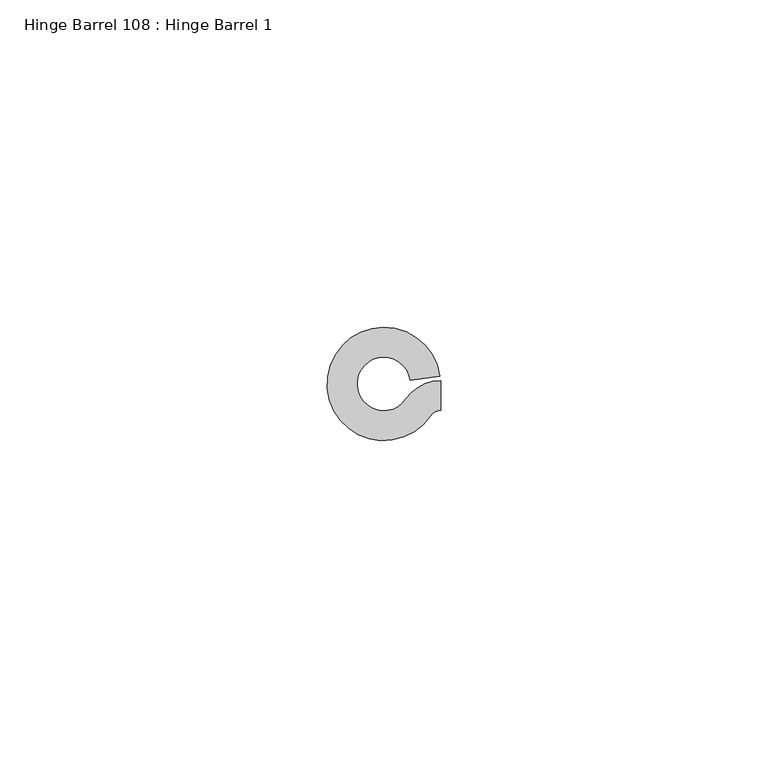
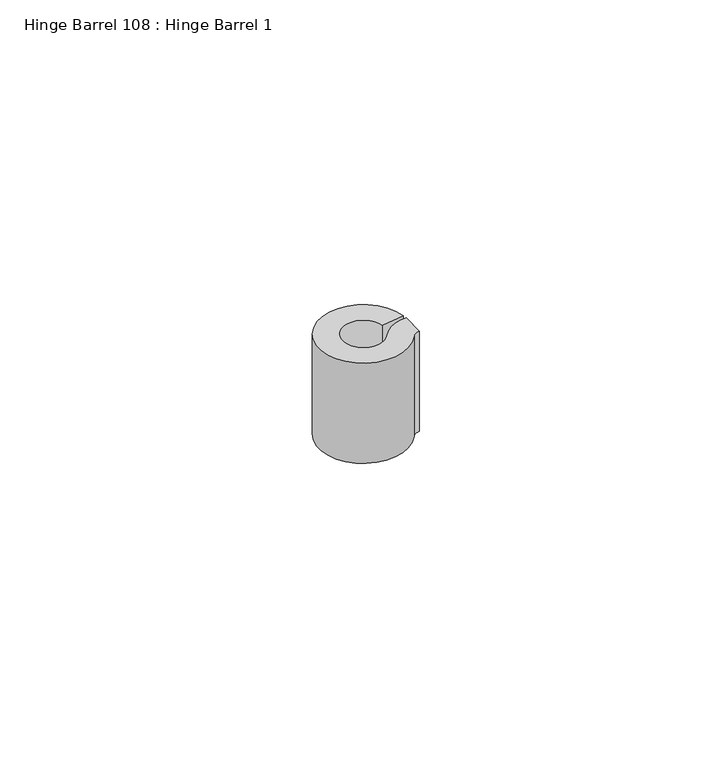
"""IFC4 building model written with IfcOpenShell, lengths in millimetres: proxy geometry, Hinge Barrel 108 : Hinge Barrel 1."""

from ifc_helpers import new_model, si_unit, point, frame, frame_2d, origin, place, context, project, spatial, polyline, circle_curve, trimmed, segment, composite_curve, outline, extrude, source, transform, mapped, element, save


def hinge_barrel_108_hinge_barrel_1_4bd796ae(model_context):
    return source(origin(), model_context, "Body", "SweptSolid", [
        extrude(outline(composite_curve([segment(trimmed(circle_curve(frame_2d((587327.8245257, -533990.5568067)), 6.4044851), [point((587322.5194669, -533986.9688017))], [point((587327.8245257, -533984.1523216))], False, "CARTESIAN"), True, "CONTINUOUS"), segment(polyline([(587327.8245257, -533984.1523216), (587327.8245257, -533988.7163841)]), True, "CONTINUOUS"), segment(trimmed(circle_curve(frame_2d((587327.8245257, -533990.5568067)), 1.8404226), [point((587327.8245257, -533988.7163841))], [point((587326.3000393, -533989.5257409))], True, "CARTESIAN"), True, "CONTINUOUS"), segment(trimmed(circle_curve(frame_2d((587319.1320739, -533984.6777841)), 8.6534625), [point((587326.3000393, -533989.5257409))], [point((587327.7022899, -533983.4803654))], False, "CARTESIAN"), True, "CONTINUOUS"), segment(polyline([(587327.7022899, -533983.4803654), (587323.1821338, -533984.1119153)]), True, "CONTINUOUS"), segment(trimmed(circle_curve(frame_2d((587319.1320739, -533984.6777841)), 4.0894), [point((587323.1821338, -533984.1119153))], [point((587322.5194669, -533986.9688017))], True, "CARTESIAN"), True, "CONTINUOUS")], self_intersect=False)), frame((0.0, 0.0, 1250.95), z_axis=(0.0, 0.0, 1.0), x_axis=(1.0, 0.0, 0.0)), (0.0, 0.0, 1.0), 20.8359375),
    ])


if __name__ == "__main__":
    model = new_model("IFC4")
    model_context = context("Model", 3, world=origin())
    ifc_project = project(units=[si_unit("LENGTHUNIT", "METRE", prefix="MILLI")], contexts=[model_context])
    site = spatial("IfcSite", under=ifc_project)
    building = spatial("IfcBuilding", under=site)
    placement = place(None, origin())
    hinge_barrel_108_hinge_barrel_1_shape = hinge_barrel_108_hinge_barrel_1_4bd796ae(model_context)
    element("IfcBuildingElementProxy", 1, Name="Hinge Barrel 108 : Hinge Barrel 1", ObjectType="Hinge Barrel 108 : Hinge Barrel 1", at=placement, inside=building, context=model_context, shape_type="MappedRepresentation", body=[
        mapped(hinge_barrel_108_hinge_barrel_1_shape, transform((0.0, 0.0, 0.0), x_axis=(1.0, 0.0, 0.0), y_axis=(0.0, 1.0, 0.0), z_axis=(0.0, 0.0, 1.0))),
    ])
    save(model, "model.ifc")

# Revit data of these elements
# Element 1 (IfcBuildingElementProxy, "Hinge Barrel 108 : Hinge Barrel 1")
#   Materials on its faces: "6\"X6\" WELD-ON STL BUTT HINGE"
# Materials
#   "6\"X6\" WELD-ON STL BUTT HINGE": class "Metal", colour RGB 189 187 185, transparency 0, Description = "Carbon steel", Cost = 0
